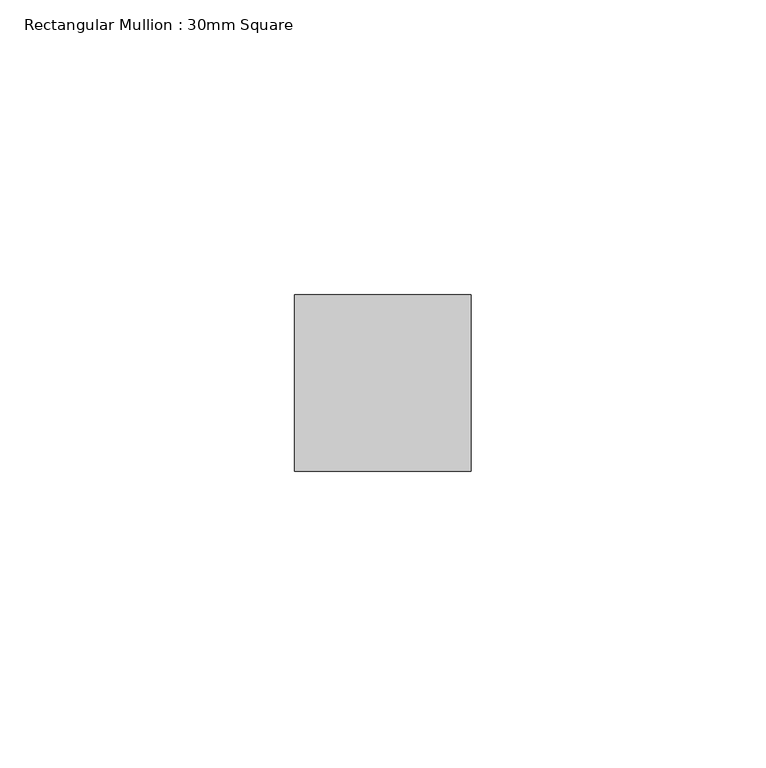
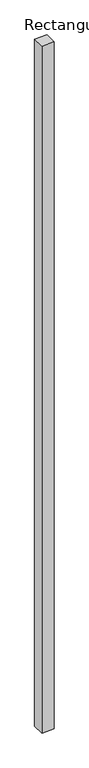
"""IFC4 building model written with IfcOpenShell, lengths in millimetres: member geometry, Rectangular Mullion : 30mm Square."""

from ifc_helpers import new_model, si_unit, frame, origin, place, context, project, spatial, polyline, outline, extrude, source, transform, mapped, element, save


def rectangular_mullion_30mm_square_281b7b6d(model_context):
    return source(origin(), model_context, "Body", "SweptSolid", [
        extrude(outline(polyline([(15.0, 15.0), (15.0, -15.0), (-15.0, -15.0), (-15.0, 15.0), (15.0, 15.0)])), frame((0.0, 0.0, -1763.4174675), z_axis=(0.0, 0.0, 1.0), x_axis=(1.0, 0.0, 0.0)), (0.0, 0.0, 1.0), 1763.4174675),
    ])


if __name__ == "__main__":
    model = new_model("IFC4")
    model_context = context("Model", 3, world=origin())
    ifc_project = project(units=[si_unit("LENGTHUNIT", "METRE", prefix="MILLI")], contexts=[model_context])
    site = spatial("IfcSite", under=ifc_project)
    building = spatial("IfcBuilding", under=site)
    placement = place(None, origin())
    rectangular_mullion_30mm_square_shape = rectangular_mullion_30mm_square_281b7b6d(model_context)
    element("IfcMember", 1, ObjectType="Rectangular Mullion : 30mm Square", at=placement, inside=building, context=model_context, shape_type="MappedRepresentation", body=[
        mapped(rectangular_mullion_30mm_square_shape, transform((0.0, 0.0, 0.0), x_axis=(1.0, 0.0, 0.0), y_axis=(0.0, 1.0, 0.0), z_axis=(0.0, 0.0, 1.0))),
    ])
    save(model, "model.ifc")

# Revit data of these elements
# Type "Rectangular Mullion : 30mm Square"
#   built-in parameter 1007304 = 0.0984252 (stored number, unit not read)
#   built-in parameter 1007301 = 0.0492126 (stored number, unit not read)
#   built-in parameter 1007300 = 0.0492126 (stored number, unit not read)
# Element 1 (IfcMember, "Rectangular Mullion : 30mm Square")
#   Materials on its faces: "Aluminum"
# Materials
#   "Aluminum": class "Metal", colour RGB 244 244 244, transparency 0, Description = "Aluminum 6061", Cost = 0
